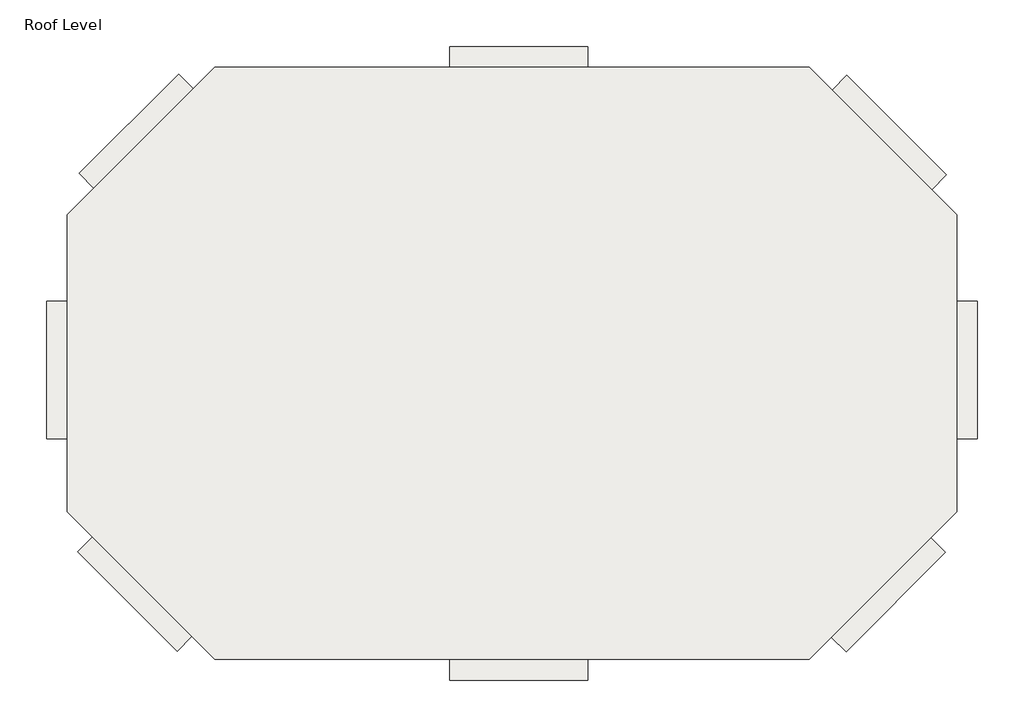
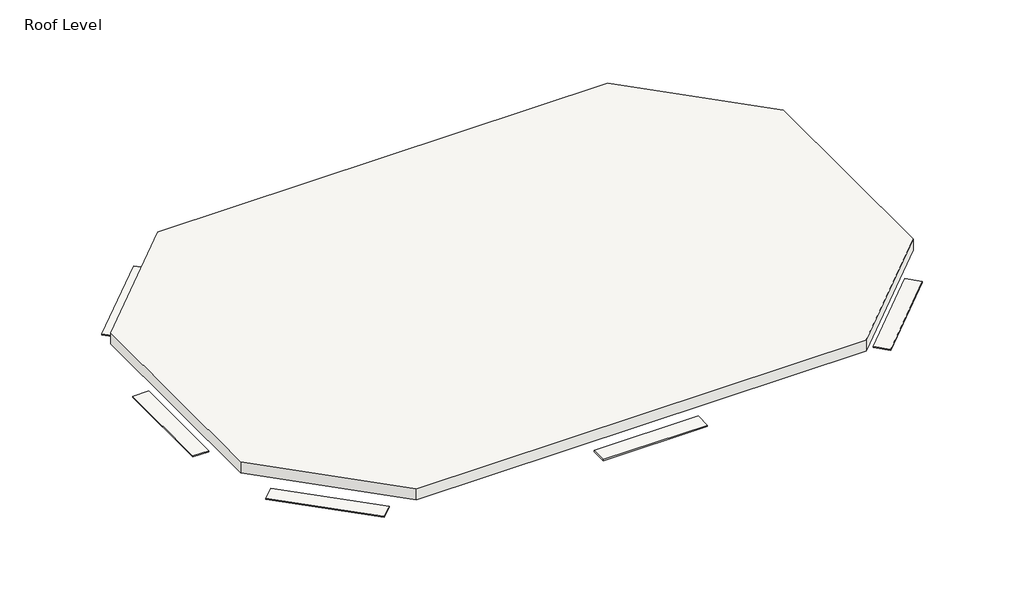
# One storey: 9 roofs.
"""IFC4 building model written with IfcOpenShell, lengths in millimetres."""

from ifc_helpers import new_model, si_unit, frame, origin, place, context, project, spatial, polyline, outline, extrude, element, save

model = new_model("IFC4")

# Units and contexts
model_context = context("Model", 3, world=origin())
ifc_project = project(units=[si_unit("LENGTHUNIT", "METRE", prefix="MILLI")], contexts=[model_context])

# Site, building, storey
site = spatial("IfcSite", under=ifc_project)
building = spatial("IfcBuilding", under=site)
storey = spatial("IfcBuildingStorey", under=building, Name="Roof Level", Elevation=7924.8)

# Roofs
placement = place(None, origin())
element("IfcRoof", 1, ObjectType="Generic - 125mm shading", at=placement, inside=storey, context=model_context, shape_type="SweptSolid", body=[
    extrude(outline(polyline([(18552.7836697, -8602.5147149), (23180.3836697, -8602.5147149), (23180.3836697, -9302.5147149), (18552.7836697, -9302.5147149), (18552.7836697, -8602.5147149)])), frame((0.0, 0.0, 7412.4), z_axis=(0.0, 0.0, 1.0), x_axis=(1.0, 0.0, 0.0)), (0.0, 0.0, 1.0), 50.0),
])
element("IfcRoof", 2, ObjectType="Generic - 125mm shading", at=placement, inside=storey, context=model_context, shape_type="SweptSolid", body=[
    extrude(outline(polyline([(23180.3836697, 11296.9802217), (18552.7836697, 11296.9802217), (18552.7836697, 11996.9802217), (23180.3836697, 11996.9802217), (23180.3836697, 11296.9802217)])), frame((0.0, 0.0, 7412.4), z_axis=(0.0, 0.0, 1.0), x_axis=(1.0, 0.0, 0.0)), (0.0, 0.0, 1.0), 50.0),
])
element("IfcRoof", 3, ObjectType="Generic - 125mm shading", at=placement, inside=storey, context=model_context, shape_type="SweptSolid", body=[
    extrude(outline(polyline([(34745.7885808, 7190.4058824), (31403.3995039, 10532.7949592), (31895.6627273, 11025.0581826), (35238.0518042, 7682.6691057), (34745.7885808, 7190.4058824)])), frame((0.0, 0.0, 7362.4), z_axis=(0.0, 0.0, 1.0), x_axis=(1.0, 0.0, 0.0)), (0.0, 0.0, 1.0), 50.0),
])
element("IfcRoof", 4, ObjectType="Generic - 125mm shading", at=placement, inside=storey, context=model_context, shape_type="SweptSolid", body=[
    extrude(outline(polyline([(31379.6986616, -7862.0302949), (34722.0877385, -4519.641218), (35214.3509618, -5011.9044414), (31871.961885, -8354.2935183), (31379.6986616, -7862.0302949)])), frame((0.0, 0.0, 7362.4), z_axis=(0.0, 0.0, 1.0), x_axis=(1.0, 0.0, 0.0)), (0.0, 0.0, 1.0), 50.0),
])
element("IfcRoof", 5, ObjectType="Generic - 125mm shading", at=placement, inside=storey, context=model_context, shape_type="SweptSolid", body=[
    extrude(outline(polyline([(9921.2320547, 10578.9980348), (6578.8429778, 7236.6089579), (6086.5797544, 7728.8721813), (9428.9688313, 11071.2612582), (9921.2320547, 10578.9980348)])), frame((0.0, 0.0, 7362.4), z_axis=(0.0, 0.0, 1.0), x_axis=(1.0, 0.0, 0.0)), (0.0, 0.0, 1.0), 50.0),
])
element("IfcRoof", 6, ObjectType="Generic - 125mm shading", at=placement, inside=storey, context=model_context, shape_type="SweptSolid", body=[
    extrude(outline(polyline([(6532.6399022, -4495.9403757), (9875.0289791, -7838.3294525), (9382.7657557, -8330.5926759), (6040.3766789, -4988.203599), (6532.6399022, -4495.9403757)])), frame((0.0, 0.0, 7362.4), z_axis=(0.0, 0.0, 1.0), x_axis=(1.0, 0.0, 0.0)), (0.0, 0.0, 1.0), 50.0),
])
element("IfcRoof", 7, ObjectType="Generic - 125mm shading", at=placement, inside=storey, context=model_context, shape_type="SweptSolid", body=[
    extrude(outline(polyline([(35588.9617098, -1191.3598794), (35588.9617098, 3436.2401206), (36288.9617098, 3436.2401206), (36288.9617098, -1191.3598794), (35588.9617098, -1191.3598794)])), frame((0.0, 0.0, 7412.4), z_axis=(0.0, 0.0, 1.0), x_axis=(1.0, 0.0, 0.0)), (0.0, 0.0, 1.0), 50.0),
])
element("IfcRoof", 8, ObjectType="Generic - 125mm shading", at=placement, inside=storey, context=model_context, shape_type="SweptSolid", body=[
    extrude(outline(polyline([(5689.4667732, 3436.2401206), (5689.4667732, -1191.3598794), (4989.4667732, -1191.3598794), (4989.4667732, 3436.2401206), (5689.4667732, 3436.2401206)])), frame((0.0, 0.0, 7412.4), z_axis=(0.0, 0.0, 1.0), x_axis=(1.0, 0.0, 0.0)), (0.0, 0.0, 1.0), 50.0),
])
element("IfcRoof", 9, ObjectType="Pitched - Warm - Industrial", at=placement, inside=storey, context=model_context, shape_type="SweptSolid", body=[
    extrude(outline(polyline([(5689.4667732, 6347.2327534), (10639.2142415, 11296.9802217), (30639.2142415, 11296.9802217), (35588.9617098, 6347.2327534), (35588.9617098, -3652.7672466), (30639.2142415, -8602.5147149), (10639.2142415, -8602.5147149), (5689.4667732, -3652.7672466), (5689.4667732, 6347.2327534)])), frame((0.0, 0.0, 7924.8), z_axis=(0.0, 0.0, 1.0), x_axis=(1.0, 0.0, 0.0)), (0.0, 0.0, 1.0), 515.0),
])

save(model, "model.ifc")

# Revit data of these elements
# Type "Generic - 125mm shading"
#   Layers, outside or top first: 50 mm no material (function 1)
# Type "Pitched - Warm - Industrial"
#   Layers, outside or top first: 50 mm "Roofing, Standing Seam" (function 5); 220 mm "Rigid insulation" (function 3); 20 mm "Metal Panel" (function 4); 225 mm "Steel Purlins" (function 1)
# Elements 1, 2, 7, 8 (IfcRoof, "Generic - 125mm shading")
#   built-in parameter 1001705 = 24.4829 (stored number, unit not read)
#   built-in parameter 1001701 = -1.6811 (stored number, unit not read)
#   built-in parameter 1001710 = 33615
#   Phase Created = New Construction
#   Materials on its faces: "Default Roof"
# Elements 3, 4, 5, 6 (IfcRoof, "Generic - 125mm shading")
#   built-in parameter 1001705 = 24.3189 (stored number, unit not read)
#   built-in parameter 1001701 = -1.84514 (stored number, unit not read)
#   built-in parameter 1001710 = 33615
#   Phase Created = New Construction
#   Materials on its faces: "Default Roof"
# Element 9 (IfcRoof, "Pitched - Warm - Industrial")
#   built-in parameter 1001705 = 27.6896 (stored number, unit not read)
#   built-in parameter 1001710 = 33615
#   Phase Created = New Construction
#   Materials on its faces: "Steel Purlins", "Roofing, Standing Seam"
# Materials
#   "Roofing, Standing Seam": class "Metal", colour RGB 247 247 247, transparency 0, Description = "Aluminum standing seam roofing", Cost = 0
#   "Rigid insulation": class "Generic", colour RGB 127 127 127, transparency 0, Description = "Rigid foam insulation board", Cost = 0
#   "Metal Panel": class "Metal", colour RGB 247 247 247, transparency 0, Description = "Stainless steel panels", Cost = 0
#   "Steel Purlins": class "Metal", colour RGB 247 247 247, transparency 0, Description = "Light gauge steel purlins", Cost = 0
#   "Default Roof": class "Miscellaneous", colour RGB 0 127 0, transparency 0, Cost = 0
